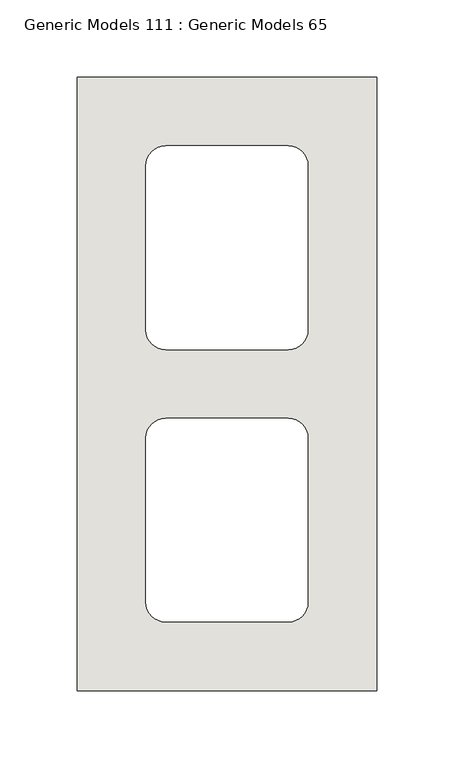
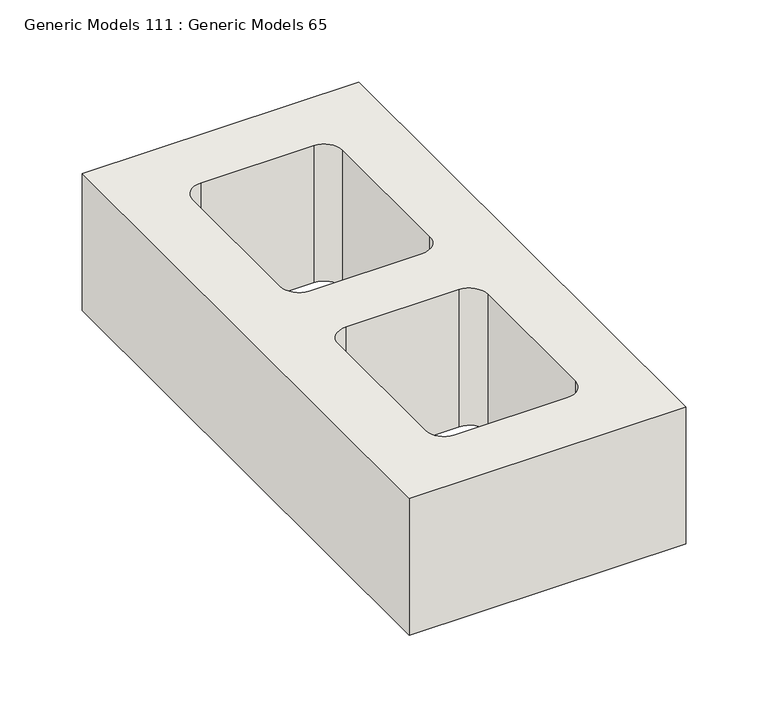
"""IFC4 building model written with IfcOpenShell, lengths in millimetres: wall geometry, Generic Models 111 : Generic Models 65."""

from ifc_helpers import new_model, si_unit, point, frame, frame_2d, origin, place, context, project, spatial, polyline, circle_curve, trimmed, segment, composite_curve, outline, extrude, source, transform, mapped, element, save


def generic_models_111_generic_models_65_cd3c3018(model_context):
    return source(origin(), model_context, "Body", "SweptSolid", [
        extrude(outline(polyline([(373607.0125, 292.1), (373413.3375, 292.1), (373413.3375, 688.975), (373607.0125, 688.975), (373607.0125, 292.1)]), holes=[composite_curve([segment(polyline([(373562.5625, 525.4625), (373562.5625, 631.825)]), True, "CONTINUOUS"), segment(trimmed(circle_curve(frame_2d((373549.8625, 631.825)), 12.7), [point((373562.5625, 631.825))], [point((373549.8625, 644.525))], True, "CARTESIAN"), True, "CONTINUOUS"), segment(polyline([(373549.8625, 644.525), (373470.4875, 644.525)]), True, "CONTINUOUS"), segment(trimmed(circle_curve(frame_2d((373470.4875, 631.825)), 12.7), [point((373470.4875, 644.525))], [point((373457.7875, 631.825))], True, "CARTESIAN"), True, "CONTINUOUS"), segment(polyline([(373457.7875, 631.825), (373457.7875, 525.4625)]), True, "CONTINUOUS"), segment(trimmed(circle_curve(frame_2d((373470.4875, 525.4625)), 12.7), [point((373457.7875, 525.4625))], [point((373470.4875, 512.7625))], True, "CARTESIAN"), True, "CONTINUOUS"), segment(polyline([(373470.4875, 512.7625), (373549.8625, 512.7625)]), True, "CONTINUOUS"), segment(trimmed(circle_curve(frame_2d((373549.8625, 525.4625)), 12.7), [point((373549.8625, 512.7625))], [point((373562.5625, 525.4625))], True, "CARTESIAN"), True, "CONTINUOUS")], self_intersect=False), composite_curve([segment(polyline([(373457.7875, 455.6125), (373457.7875, 349.25)]), True, "CONTINUOUS"), segment(trimmed(circle_curve(frame_2d((373470.4875, 349.25)), 12.7), [point((373457.7875, 349.25))], [point((373470.4875, 336.55))], True, "CARTESIAN"), True, "CONTINUOUS"), segment(polyline([(373470.4875, 336.55), (373549.8625, 336.55)]), True, "CONTINUOUS"), segment(trimmed(circle_curve(frame_2d((373549.8625, 349.25)), 12.7), [point((373549.8625, 336.55))], [point((373562.5625, 349.25))], True, "CARTESIAN"), True, "CONTINUOUS"), segment(polyline([(373562.5625, 349.25), (373562.5625, 455.6125)]), True, "CONTINUOUS"), segment(trimmed(circle_curve(frame_2d((373549.8625, 455.6125)), 12.7), [point((373562.5625, 455.6125))], [point((373549.8625, 468.3125))], True, "CARTESIAN"), True, "CONTINUOUS"), segment(polyline([(373549.8625, 468.3125), (373470.4875, 468.3125)]), True, "CONTINUOUS"), segment(trimmed(circle_curve(frame_2d((373470.4875, 455.6125)), 12.7), [point((373470.4875, 468.3125))], [point((373457.7875, 455.6125))], True, "CARTESIAN"), True, "CONTINUOUS")], self_intersect=False)]), frame((0.0, 0.0, 2438.3999999), z_axis=(0.0, 0.0, 1.0), x_axis=(1.0, 0.0, 0.0)), (0.0, 0.0, 1.0), 101.6000001),
    ])


if __name__ == "__main__":
    model = new_model("IFC4")
    model_context = context("Model", 3, world=origin())
    ifc_project = project(units=[si_unit("LENGTHUNIT", "METRE", prefix="MILLI")], contexts=[model_context])
    site = spatial("IfcSite", under=ifc_project)
    building = spatial("IfcBuilding", under=site)
    placement = place(None, origin())
    generic_models_111_generic_models_65_shape = generic_models_111_generic_models_65_cd3c3018(model_context)
    element("IfcWall", 1, ObjectType="Generic Models 111 : Generic Models 65", at=placement, inside=building, context=model_context, shape_type="MappedRepresentation", body=[
        mapped(generic_models_111_generic_models_65_shape, transform((0.0, 0.0, 0.0), x_axis=(1.0, 0.0, 0.0), y_axis=(0.0, 1.0, 0.0), z_axis=(0.0, 0.0, 1.0))),
    ])
    save(model, "model.ifc")

# Revit data of these elements
# Element 1 (IfcWall, "Generic Models 111 : Generic Models 65")
#   Materials on its faces: "CMU (SEE 'WALL TAG' FOR SIZE)"
# Materials
#   "CMU (SEE 'WALL TAG' FOR SIZE)": class "Masonry", colour RGB 203 203 199, transparency 0, Description = "Concrete masonry units", Cost = 0
